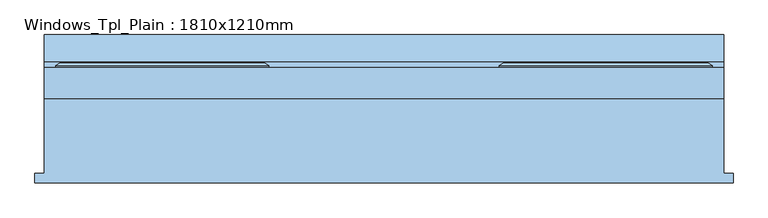
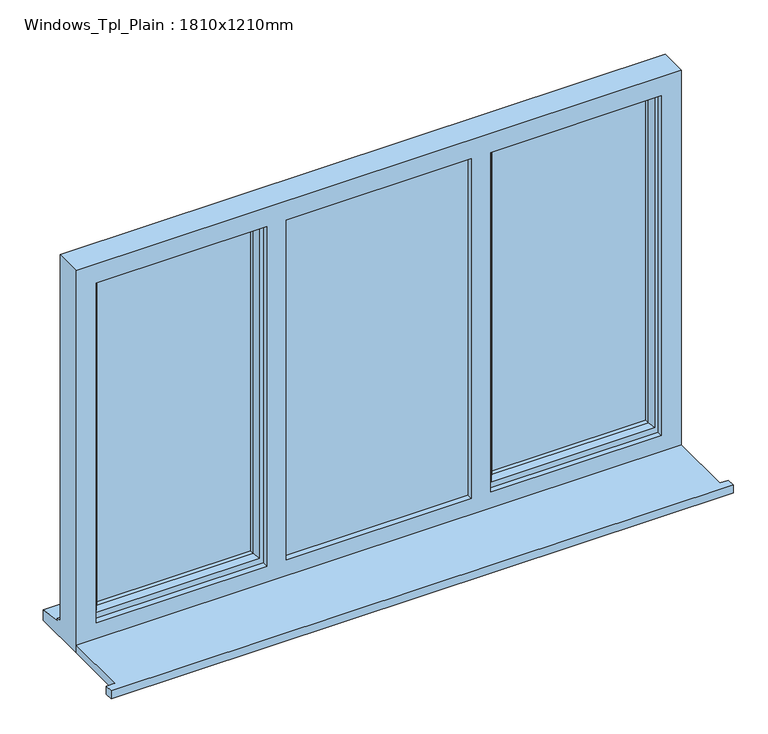
"""IFC4 building model written with IfcOpenShell, lengths in millimetres: window geometry, Windows_Tpl_Plain : 1810x1210mm."""

from ifc_helpers import new_model, si_unit, frame, origin, place, context, project, spatial, polyline, outline, extrude, faceted_brep, source, transform, mapped, element, save


def windows_tpl_plain_1810x1210mm_b4f2050b(model_context):
    return source(origin(), model_context, "Body", "SolidModel", [
        extrude(outline(polyline([(-1506.6666667, -182.7934322), (-1506.6666667, -157.7934322), (-1481.6666667, -157.7934322), (-1481.6666667, 41.7065678), (328.3333333, 41.7065678), (328.3333333, -157.7934322), (353.3333333, -157.7934322), (353.3333333, -182.7934322), (-1506.6666667, -182.7934322)])), frame((0.0, 0.0, 900.0), z_axis=(0.0, 0.0, 1.0), x_axis=(1.0, 0.0, 0.0)), (0.0, 0.0, 1.0), 25.0),
        extrude(outline(polyline([(258.3333333, 88.7065678), (-230.0, 88.7065678), (-230.0, 112.7065678), (258.3333333, 112.7065678), (258.3333333, 88.7065678)])), frame((0.0, 0.0, 993.0), z_axis=(0.0, 0.0, 1.0), x_axis=(1.0, 0.0, 0.0)), (0.0, 0.0, 1.0), 1047.0),
        extrude(outline(polyline([(-863.3333333, 83.7065678), (-290.0, 83.7065678), (-290.0, 59.7065678), (-863.3333333, 59.7065678), (-863.3333333, 83.7065678)])), frame((0.0, 0.0, 963.0), z_axis=(0.0, 0.0, 1.0), x_axis=(1.0, 0.0, 0.0)), (0.0, 0.0, 1.0), 1107.0),
        extrude(outline(polyline([(-923.3333333, 88.7065678), (-1411.6666667, 88.7065678), (-1411.6666667, 112.7065678), (-923.3333333, 112.7065678), (-923.3333333, 88.7065678)])), frame((0.0, 0.0, 993.0), z_axis=(0.0, 0.0, 1.0), x_axis=(1.0, 0.0, 0.0)), (0.0, 0.0, 1.0), 1047.0),
        faceted_brep([(328.3333333, 41.7065678, 2110.0), (-1481.6666667, 41.7065678, 2110.0), (-1481.6666667, 41.7065678, 900.0), (328.3333333, 41.7065678, 900.0), (268.3333333, 41.7065678, 2050.0), (268.3333333, 41.7065678, 975.0), (-242.0, 41.7065678, 975.0), (-242.0, 41.7065678, 2050.0), (-300.0, 41.7065678, 2050.0), (-300.0, 41.7065678, 975.0), (-853.3333333, 41.7065678, 975.0), (-853.3333333, 41.7065678, 2050.0), (-911.3333333, 41.7065678, 2050.0), (-911.3333333, 41.7065678, 975.0), (-1421.6666667, 41.7065678, 975.0), (-1421.6666667, 41.7065678, 2050.0), (-1481.6666667, 124.7065678, 2110.0), (-1481.6666667, 124.7065678, 951.0), (-1481.6666667, 139.7065678, 949.68767), (-1481.6666667, 139.7065678, 944.7449676), (-1481.6666667, 212.2065678, 933.8088847), (-1481.6666667, 212.2065678, 900.0), (328.3333333, 124.7065678, 2110.0), (328.3333333, 124.7065678, 951.0), (-1441.6666667, 124.7065678, 2070.0), (-1441.6666667, 124.7065678, 963.0), (-893.3333333, 124.7065678, 963.0), (-893.3333333, 124.7065678, 2070.0), (-853.3333333, 124.7065678, 2070.0), (-853.3333333, 124.7065678, 963.0), (-300.0, 124.7065678, 963.0), (-300.0, 124.7065678, 2070.0), (-260.0, 124.7065678, 2070.0), (-260.0, 124.7065678, 963.0), (288.3333333, 124.7065678, 963.0), (288.3333333, 124.7065678, 2070.0), (-1441.6666667, 59.7065678, 2070.0), (-1441.6666667, 59.7065678, 963.0), (-863.3333333, 59.7065678, 2070.0), (-290.0, 59.7065678, 2070.0), (-290.0, 59.7065678, 963.0), (-863.3333333, 59.7065678, 963.0), (-300.0, 59.7065678, 2050.0), (-853.3333333, 59.7065678, 2050.0), (-853.3333333, 59.7065678, 975.0), (-300.0, 59.7065678, 975.0), (-260.0, 59.7065678, 2070.0), (288.3333333, 59.7065678, 2070.0), (288.3333333, 59.7065678, 963.0), (-260.0, 59.7065678, 963.0), (268.3333333, 59.7065678, 2050.0), (-242.0, 59.7065678, 2050.0), (-242.0, 59.7065678, 975.0), (268.3333333, 59.7065678, 975.0), (-893.3333333, 59.7065678, 2070.0), (-893.3333333, 59.7065678, 963.0), (-911.3333333, 59.7065678, 2050.0), (-1421.6666667, 59.7065678, 2050.0), (-1421.6666667, 59.7065678, 975.0), (-911.3333333, 59.7065678, 975.0), (-853.3333333, 83.7065678, 2070.0), (-300.0, 83.7065678, 2070.0), (-290.0, 83.7065678, 2070.0), (-863.3333333, 83.7065678, 2070.0), (328.3333333, 212.2065678, 900.0), (328.3333333, 212.2065678, 933.8088847), (328.3333333, 139.7065678, 944.7449676), (328.3333333, 139.7065678, 949.68767), (-853.3333333, 83.7065678, 963.0), (-863.3333333, 83.7065678, 963.0), (-290.0, 83.7065678, 963.0), (-300.0, 83.7065678, 963.0)], [[[0, 1, 2, 3], [4, 5, 6, 7], [8, 9, 10, 11], [12, 13, 14, 15]], [[2, 1, 16, 17, 18, 19, 20, 21]], [[17, 16, 22, 23], [24, 25, 26, 27], [28, 29, 30, 31], [32, 33, 34, 35]], [[25, 24, 36, 37]], [[38, 39, 40, 41], [42, 43, 44, 45]], [[46, 47, 48, 49], [50, 51, 52, 53]], [[36, 54, 55, 37], [56, 57, 58, 59]], [[57, 15, 14, 58]], [[1, 0, 22, 16]], [[36, 24, 27, 54]], [[35, 47, 46, 32]], [[60, 28, 31, 61, 62, 39, 38, 63]], [[15, 57, 56, 12]], [[50, 4, 7, 51]], [[11, 43, 42, 8]], [[23, 22, 0, 3, 64, 65, 66, 67]], [[35, 34, 48, 47]], [[4, 50, 53, 5]], [[43, 11, 10, 44]], [[12, 56, 59, 13]], [[27, 26, 55, 54]], [[29, 28, 60, 68]], [[68, 60, 63, 69]], [[69, 63, 38, 41]], [[62, 70, 40, 39]], [[70, 62, 61, 71]], [[71, 61, 31, 30]], [[33, 32, 46, 49]], [[51, 7, 6, 52]], [[8, 42, 45, 9]], [[64, 3, 2, 21]], [[65, 64, 21, 20]], [[66, 65, 20, 19]], [[67, 66, 19, 18]], [[23, 67, 18, 17]], [[26, 25, 37, 55]], [[34, 33, 49, 48]], [[41, 40, 70, 71, 30, 29, 68, 69]], [[6, 5, 53, 52]], [[45, 44, 10, 9]], [[59, 58, 14, 13]]]),
        faceted_brep([(-883.3333333, 124.7065678, 2080.0), (-883.3333333, 130.4800705, 2080.0), (-1451.6666667, 130.4800705, 2080.0), (-1451.6666667, 124.7065678, 2080.0), (-893.3333333, 59.7065678, 2070.0), (-893.3333333, 124.7065678, 2070.0), (-1441.6666667, 124.7065678, 2070.0), (-1441.6666667, 59.7065678, 2070.0), (-933.3333333, 74.1994677, 2030.0), (-923.1852956, 59.7065678, 2040.1480377), (-1411.8147044, 59.7065678, 2040.1480377), (-1401.6666667, 74.1994677, 2030.0), (-933.3333333, 88.7065678, 2030.0), (-1401.6666667, 88.7065678, 2030.0), (-923.3333333, 112.7065678, 2040.0), (-923.3333333, 88.7065678, 2040.0), (-1411.6666667, 88.7065678, 2040.0), (-1411.6666667, 112.7065678, 2040.0), (-933.3333333, 130.4800705, 2030.0), (-933.3333333, 112.7065678, 2030.0), (-1401.6666667, 112.7065678, 2030.0), (-1401.6666667, 130.4800705, 2030.0), (-914.5187677, 136.2535732, 2048.8145656), (-1420.4812323, 136.2535732, 2048.8145656), (-894.964114, 136.2535732, 2068.3692194), (-1440.035886, 136.2535732, 2068.3692194), (-1451.6666667, 130.4800705, 953.0), (-1451.6666667, 124.7065678, 953.0), (-1441.6666667, 124.7065678, 963.0), (-1441.6666667, 59.7065678, 963.0), (-1411.8147044, 59.7065678, 992.8519623), (-1401.6666667, 74.1994677, 1003.0), (-1401.6666667, 88.7065678, 1003.0), (-1411.6666667, 88.7065678, 993.0), (-1411.6666667, 112.7065678, 993.0), (-1401.6666667, 112.7065678, 1003.0), (-1401.6666667, 130.4800705, 1003.0), (-1420.4812323, 136.2535732, 984.1854344), (-1440.035886, 136.2535732, 964.6307806), (-883.3333333, 130.4800705, 953.0), (-883.3333333, 124.7065678, 953.0), (-893.3333333, 124.7065678, 963.0), (-893.3333333, 59.7065678, 963.0), (-923.1852956, 59.7065678, 992.8519623), (-933.3333333, 74.1994677, 1003.0), (-933.3333333, 88.7065678, 1003.0), (-923.3333333, 88.7065678, 993.0), (-923.3333333, 112.7065678, 993.0), (-933.3333333, 112.7065678, 1003.0), (-933.3333333, 130.4800705, 1003.0), (-914.5187677, 136.2535732, 984.1854344), (-894.964114, 136.2535732, 964.6307806)], [[[0, 1, 2, 3]], [[4, 5, 6, 7]], [[8, 9, 10, 11]], [[12, 8, 11, 13]], [[14, 15, 16, 17]], [[18, 19, 20, 21]], [[22, 18, 21, 23]], [[1, 24, 25, 2]], [[3, 2, 26, 27]], [[7, 6, 28, 29]], [[11, 10, 30, 31]], [[13, 11, 31, 32]], [[17, 16, 33, 34]], [[21, 20, 35, 36]], [[23, 21, 36, 37]], [[2, 25, 38, 26]], [[27, 26, 39, 40]], [[0, 3, 27, 40], [41, 28, 6, 5]], [[29, 28, 41, 42]], [[4, 7, 29, 42], [43, 30, 10, 9]], [[31, 30, 43, 44]], [[32, 31, 44, 45]], [[46, 33, 16, 15], [12, 13, 32, 45]], [[34, 33, 46, 47]], [[14, 17, 34, 47], [48, 35, 20, 19]], [[36, 35, 48, 49]], [[37, 36, 49, 50]], [[51, 38, 25, 24], [22, 23, 37, 50]], [[26, 38, 51, 39]], [[40, 39, 1, 0]], [[42, 41, 5, 4]], [[44, 43, 9, 8]], [[45, 44, 8, 12]], [[47, 46, 15, 14]], [[49, 48, 19, 18]], [[50, 49, 18, 22]], [[39, 51, 24, 1]]]),
        faceted_brep([(-270.0, 124.7065678, 2080.0), (-270.0, 130.4800705, 2080.0), (-270.0, 130.4800705, 953.0), (-270.0, 124.7065678, 953.0), (-260.0, 59.7065678, 2070.0), (-260.0, 124.7065678, 2070.0), (-260.0, 124.7065678, 963.0), (-260.0, 59.7065678, 963.0), (-220.0, 74.1994677, 2030.0), (-230.1480377, 59.7065678, 2040.1480377), (-230.1480377, 59.7065678, 992.8519623), (-220.0, 74.1994677, 1003.0), (-220.0, 88.7065678, 2030.0), (-220.0, 88.7065678, 1003.0), (-230.0, 112.7065678, 2040.0), (-230.0, 88.7065678, 2040.0), (-230.0, 88.7065678, 993.0), (-230.0, 112.7065678, 993.0), (-220.0, 130.4800705, 2030.0), (-220.0, 112.7065678, 2030.0), (-220.0, 112.7065678, 1003.0), (-220.0, 130.4800705, 1003.0), (-237.4457548, 136.2535732, 2047.4457548), (-237.4457548, 136.2535732, 985.5542452), (-259.2153903, 136.2535732, 2069.2153903), (-259.2153903, 136.2535732, 963.7846097), (298.3333333, 130.4800705, 953.0), (298.3333333, 124.7065678, 953.0), (288.3333333, 124.7065678, 963.0), (288.3333333, 59.7065678, 963.0), (258.4813711, 59.7065678, 992.8519623), (248.3333333, 74.1994677, 1003.0), (248.3333333, 88.7065678, 1003.0), (258.3333333, 88.7065678, 993.0), (258.3333333, 112.7065678, 993.0), (248.3333333, 112.7065678, 1003.0), (248.3333333, 130.4800705, 1003.0), (265.7790881, 136.2535732, 985.5542452), (287.5487236, 136.2535732, 963.7846097), (298.3333333, 130.4800705, 2080.0), (298.3333333, 124.7065678, 2080.0), (288.3333333, 124.7065678, 2070.0), (288.3333333, 59.7065678, 2070.0), (258.4813711, 59.7065678, 2040.1480377), (248.3333333, 74.1994677, 2030.0), (248.3333333, 88.7065678, 2030.0), (258.3333333, 88.7065678, 2040.0), (258.3333333, 112.7065678, 2040.0), (248.3333333, 112.7065678, 2030.0), (248.3333333, 130.4800705, 2030.0), (265.7790881, 136.2535732, 2047.4457548), (287.5487236, 136.2535732, 2069.2153903)], [[[0, 1, 2, 3]], [[4, 5, 6, 7]], [[8, 9, 10, 11]], [[12, 8, 11, 13]], [[14, 15, 16, 17]], [[18, 19, 20, 21]], [[22, 18, 21, 23]], [[1, 24, 25, 2]], [[3, 2, 26, 27]], [[7, 6, 28, 29]], [[11, 10, 30, 31]], [[13, 11, 31, 32]], [[17, 16, 33, 34]], [[21, 20, 35, 36]], [[23, 21, 36, 37]], [[2, 25, 38, 26]], [[27, 26, 39, 40]], [[29, 28, 41, 42]], [[31, 30, 43, 44]], [[32, 31, 44, 45]], [[34, 33, 46, 47]], [[36, 35, 48, 49]], [[37, 36, 49, 50]], [[26, 38, 51, 39]], [[40, 39, 1, 0]], [[3, 27, 40, 0], [5, 41, 28, 6]], [[42, 41, 5, 4]], [[7, 29, 42, 4], [9, 43, 30, 10]], [[44, 43, 9, 8]], [[45, 44, 8, 12]], [[15, 46, 33, 16], [13, 32, 45, 12]], [[47, 46, 15, 14]], [[17, 34, 47, 14], [19, 48, 35, 20]], [[49, 48, 19, 18]], [[50, 49, 18, 22]], [[24, 51, 38, 25], [23, 37, 50, 22]], [[39, 51, 24, 1]]]),
    ])


if __name__ == "__main__":
    model = new_model("IFC4")
    model_context = context("Model", 3, world=origin())
    ifc_project = project(units=[si_unit("LENGTHUNIT", "METRE", prefix="MILLI")], contexts=[model_context])
    site = spatial("IfcSite", under=ifc_project)
    building = spatial("IfcBuilding", under=site)
    placement = place(None, origin())
    windows_tpl_plain_1810x1210mm_shape = windows_tpl_plain_1810x1210mm_b4f2050b(model_context)
    element("IfcWindow", 1, ObjectType="Windows_Tpl_Plain : 1810x1210mm", at=placement, inside=building, context=model_context, shape_type="MappedRepresentation", body=[
        mapped(windows_tpl_plain_1810x1210mm_shape, transform((0.0, 0.0, 0.0), x_axis=(1.0, 0.0, 0.0), y_axis=(0.0, 1.0, 0.0), z_axis=(0.0, 0.0, 1.0))),
    ])
    save(model, "model.ifc")

# Revit data of these elements
# Type "Windows_Tpl_Plain : 1810x1210mm"
#   Type Mark = "79"
#   Operation = "TriplePanelVertical"
#   Construction Type Id = "GSP4R"
#   Manufacturer = "Revit"
#   Keynote = "L10"
#   Analytic Construction = "1/8 in Pilkington single glazing"
#   Wrap Layers (Ext) from Ext = 102.5 mm
#   Wrap Layers (Int) from Ext = 177.5 mm
#   Window Board Projection = 25 mm
#   Window Board Extension = 25 mm
#   Visual Light Transmittance = 0.9
#   Solar Heat Gain Coefficient = 0.78
#   Rough Width = 1810 mm
#   Rough Height = 1210 mm
#   Height = 1210 mm
#   Width = 1810 mm
#   Heat Transfer Coefficient (U) = 3.6886 W/(m²·K)
#   Glazing Thickness = 24 mm
#   FrameOffset - External = 50 mm
#   Frame Depth = 65 mm
#   Default Head Height = 2110 mm
#   Cill Depth = 87.5 mm
#   Cavity Closer Width = 50 mm
#   Cavity Closer Offset from Ext = 102.5 mm
#   Cavity Closer Depth = 85 mm
#   Vis - Cavity Closers = yes
#   Define Thermal Properties by = 1
#   Material Trim = Window Frame
#   Material Glass = Glass
#   Material Frame = Window Frame
#   Wall Closure = (empty or 0)
# Element 1 (IfcWindow, "Windows_Tpl_Plain : 1810x1210mm")
#   Materials on its faces: "Window Frame", "Glass"
# Materials
#   "Window Frame": class "Miscellaneous", colour RGB 249 249 249, transparency 0, Keynote = "L10"
#   "Glass": class "Glass", colour RGB 0 128 192, transparency 0.9, Description = "Soda Lime Glass", Cost = 0
